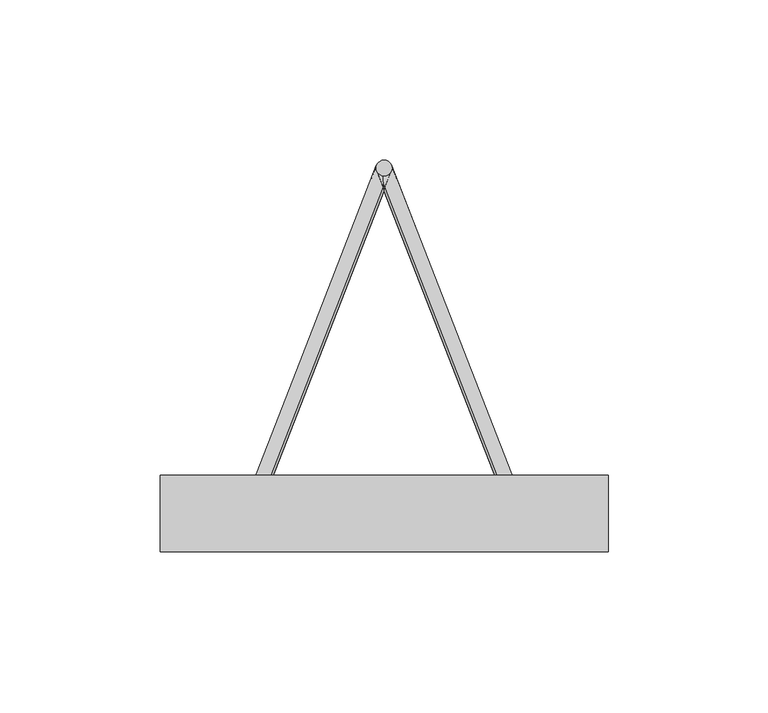
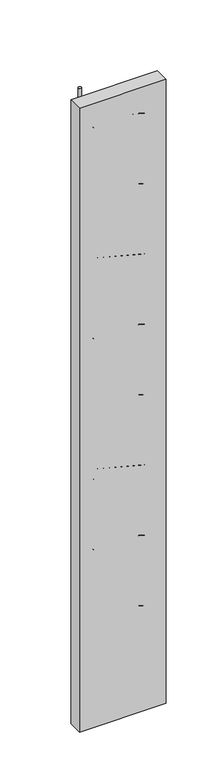
"""IFC4 building model written with IfcOpenShell, lengths in millimetres: proxy geometry, Vigota 4 (Pano 6) (Mf = 85)."""

from ifc_helpers import new_model, si_unit, point, frame, frame_2d, origin, origin_with_axes, origin_2d, place, context, project, spatial, polyline, circle_curve, trimmed, segment, composite_curve, outline, extrude, source, transform, mapped, element, save


def structural_framing_46c3b547(model_context):
    return source(origin(), model_context, "Body", "SweptSolid", [
        extrude(outline(polyline([(-70.0, 12.0), (70.0, 12.0), (70.0, -12.0), (-70.0, -12.0), (-70.0, 12.0)])), origin_with_axes(), (0.0, 0.0, 1.0), 1065.0),
        extrude(outline(composite_curve([segment(trimmed(circle_curve(frame_2d((42.0, 0.0)), 2.5), [point((44.5, 0.0))], [point((39.5, 0.0))], False, "CARTESIAN"), True, "CONTINUOUS"), segment(trimmed(circle_curve(frame_2d((42.0, 0.0)), 2.5), [point((39.5, 0.0))], [point((44.5, 0.0))], False, "CARTESIAN"), True, "CONTINUOUS")], self_intersect=False)), frame((0.0, 0.0, 28.0), z_axis=(0.0, 0.0, 1.0), x_axis=(1.0, 0.0, 0.0)), (0.0, 0.0, 1.0), 1009.0),
        extrude(outline(composite_curve([segment(trimmed(circle_curve(frame_2d((0.0, 108.0)), 2.5), [point((2.5, 108.0))], [point((-2.5, 108.0))], False, "CARTESIAN"), True, "CONTINUOUS"), segment(trimmed(circle_curve(frame_2d((0.0, 108.0)), 2.5), [point((-2.5, 108.0))], [point((2.5, 108.0))], False, "CARTESIAN"), True, "CONTINUOUS")], self_intersect=False)), frame((0.0, 0.0, 62.5), z_axis=(0.0, 0.0, 1.0), x_axis=(1.0, 0.0, 0.0)), (0.0, 0.0, 1.0), 940.0),
        extrude(outline(composite_curve([segment(trimmed(circle_curve(origin_2d(), 2.5), [point((2.5, 0.0))], [point((-2.5, 0.0))], False, "CARTESIAN"), True, "CONTINUOUS"), segment(trimmed(circle_curve(origin_2d(), 2.5), [point((-2.5, 0.0))], [point((2.5, 0.0))], False, "CARTESIAN"), True, "CONTINUOUS")], self_intersect=False)), frame((42.0, 0.0, 52.5), z_axis=(-0.3218603428886276, 0.8276408817707567, 0.4598004898837537), x_axis=(0.8192319205108605, -3.936835275445103e-11, 0.5734623443750141)), (0.0, 0.0, 1.0), 130.491379),
        extrude(outline(composite_curve([segment(trimmed(circle_curve(origin_2d(), 2.5), [point((2.5, 0.0))], [point((-2.5, 0.0))], False, "CARTESIAN"), True, "CONTINUOUS"), segment(trimmed(circle_curve(origin_2d(), 2.5), [point((-2.5, 0.0))], [point((2.5, 0.0))], False, "CARTESIAN"), True, "CONTINUOUS")], self_intersect=False)), frame((0.0, 108.0, 112.5), z_axis=(0.3218603428886276, -0.8276408817707567, 0.4598004898837537), x_axis=(0.8192319205108605, -3.936835275445103e-11, -0.5734623443750141)), (0.0, 0.0, 1.0), 130.491379),
        extrude(outline(composite_curve([segment(trimmed(circle_curve(origin_2d(), 2.5), [point((2.5, 0.0))], [point((-2.5, 0.0))], False, "CARTESIAN"), True, "CONTINUOUS"), segment(trimmed(circle_curve(origin_2d(), 2.5), [point((-2.5, 0.0))], [point((2.5, 0.0))], False, "CARTESIAN"), True, "CONTINUOUS")], self_intersect=False)), frame((42.0, 0.0, 172.5), z_axis=(-0.3218603428886276, 0.8276408817707567, 0.4598004898837537), x_axis=(0.8192319205108605, -3.936835275445103e-11, 0.5734623443750141)), (0.0, 0.0, 1.0), 130.491379),
        extrude(outline(composite_curve([segment(trimmed(circle_curve(origin_2d(), 2.5), [point((2.5, 0.0))], [point((-2.5, 0.0))], False, "CARTESIAN"), True, "CONTINUOUS"), segment(trimmed(circle_curve(origin_2d(), 2.5), [point((-2.5, 0.0))], [point((2.5, 0.0))], False, "CARTESIAN"), True, "CONTINUOUS")], self_intersect=False)), frame((0.0, 108.0, 232.5), z_axis=(0.3218603428886276, -0.8276408817707567, 0.4598004898837537), x_axis=(0.8192319205108605, -3.936835275445103e-11, -0.5734623443750141)), (0.0, 0.0, 1.0), 130.491379),
        extrude(outline(composite_curve([segment(trimmed(circle_curve(origin_2d(), 2.5), [point((2.5, 0.0))], [point((-2.5, 0.0))], False, "CARTESIAN"), True, "CONTINUOUS"), segment(trimmed(circle_curve(origin_2d(), 2.5), [point((-2.5, 0.0))], [point((2.5, 0.0))], False, "CARTESIAN"), True, "CONTINUOUS")], self_intersect=False)), frame((42.0, 0.0, 292.5), z_axis=(-0.3218603428886276, 0.8276408817707567, 0.4598004898837537), x_axis=(0.8192319205108605, -3.936835275445103e-11, 0.5734623443750141)), (0.0, 0.0, 1.0), 130.491379),
        extrude(outline(composite_curve([segment(trimmed(circle_curve(origin_2d(), 2.5), [point((2.5, 0.0))], [point((-2.5, 0.0))], False, "CARTESIAN"), True, "CONTINUOUS"), segment(trimmed(circle_curve(origin_2d(), 2.5), [point((-2.5, 0.0))], [point((2.5, 0.0))], False, "CARTESIAN"), True, "CONTINUOUS")], self_intersect=False)), frame((0.0, 108.0, 352.5), z_axis=(0.3218603428886276, -0.8276408817707567, 0.4598004898837537), x_axis=(0.8192319205108605, -3.936835275445103e-11, -0.5734623443750141)), (0.0, 0.0, 1.0), 130.491379),
        extrude(outline(composite_curve([segment(trimmed(circle_curve(origin_2d(), 2.5), [point((2.5, 0.0))], [point((-2.5, 0.0))], False, "CARTESIAN"), True, "CONTINUOUS"), segment(trimmed(circle_curve(origin_2d(), 2.5), [point((-2.5, 0.0))], [point((2.5, 0.0))], False, "CARTESIAN"), True, "CONTINUOUS")], self_intersect=False)), frame((42.0, 0.0, 412.5), z_axis=(-0.3218603428886276, 0.8276408817707567, 0.4598004898837537), x_axis=(0.8192319205108605, -3.936835275445103e-11, 0.5734623443750141)), (0.0, 0.0, 1.0), 130.491379),
        extrude(outline(composite_curve([segment(trimmed(circle_curve(origin_2d(), 2.5), [point((2.5, 0.0))], [point((-2.5, 0.0))], False, "CARTESIAN"), True, "CONTINUOUS"), segment(trimmed(circle_curve(origin_2d(), 2.5), [point((-2.5, 0.0))], [point((2.5, 0.0))], False, "CARTESIAN"), True, "CONTINUOUS")], self_intersect=False)), frame((0.0, 108.0, 472.5), z_axis=(0.3218603428886276, -0.8276408817707567, 0.4598004898837537), x_axis=(0.8192319205108605, -3.936835275445103e-11, -0.5734623443750141)), (0.0, 0.0, 1.0), 130.491379),
        extrude(outline(composite_curve([segment(trimmed(circle_curve(origin_2d(), 2.5), [point((2.5, 0.0))], [point((-2.5, 0.0))], False, "CARTESIAN"), True, "CONTINUOUS"), segment(trimmed(circle_curve(origin_2d(), 2.5), [point((-2.5, 0.0))], [point((2.5, 0.0))], False, "CARTESIAN"), True, "CONTINUOUS")], self_intersect=False)), frame((42.0, 0.0, 532.5), z_axis=(-0.3218603428886276, 0.8276408817707567, 0.4598004898837537), x_axis=(0.8192319205108605, -3.936835275445103e-11, 0.5734623443750141)), (0.0, 0.0, 1.0), 130.491379),
        extrude(outline(composite_curve([segment(trimmed(circle_curve(origin_2d(), 2.5), [point((2.5, 0.0))], [point((-2.5, 0.0))], False, "CARTESIAN"), True, "CONTINUOUS"), segment(trimmed(circle_curve(origin_2d(), 2.5), [point((-2.5, 0.0))], [point((2.5, 0.0))], False, "CARTESIAN"), True, "CONTINUOUS")], self_intersect=False)), frame((0.0, 108.0, 592.5), z_axis=(0.3218603428886276, -0.8276408817707567, 0.4598004898837537), x_axis=(0.8192319205108605, -3.936835275445103e-11, -0.5734623443750141)), (0.0, 0.0, 1.0), 130.491379),
        extrude(outline(composite_curve([segment(trimmed(circle_curve(origin_2d(), 2.5), [point((2.5, 0.0))], [point((-2.5, 0.0))], False, "CARTESIAN"), True, "CONTINUOUS"), segment(trimmed(circle_curve(origin_2d(), 2.5), [point((-2.5, 0.0))], [point((2.5, 0.0))], False, "CARTESIAN"), True, "CONTINUOUS")], self_intersect=False)), frame((42.0, 0.0, 652.5), z_axis=(-0.3218603428886276, 0.8276408817707567, 0.4598004898837537), x_axis=(0.8192319205108605, -3.936835275445103e-11, 0.5734623443750141)), (0.0, 0.0, 1.0), 130.491379),
        extrude(outline(composite_curve([segment(trimmed(circle_curve(origin_2d(), 2.5), [point((2.5, 0.0))], [point((-2.5, 0.0))], False, "CARTESIAN"), True, "CONTINUOUS"), segment(trimmed(circle_curve(origin_2d(), 2.5), [point((-2.5, 0.0))], [point((2.5, 0.0))], False, "CARTESIAN"), True, "CONTINUOUS")], self_intersect=False)), frame((0.0, 108.0, 712.5), z_axis=(0.3218603428886276, -0.8276408817707567, 0.4598004898837537), x_axis=(0.8192319205108605, -3.936835275445103e-11, -0.5734623443750141)), (0.0, 0.0, 1.0), 130.491379),
        extrude(outline(composite_curve([segment(trimmed(circle_curve(origin_2d(), 2.5), [point((2.5, 0.0))], [point((-2.5, 0.0))], False, "CARTESIAN"), True, "CONTINUOUS"), segment(trimmed(circle_curve(origin_2d(), 2.5), [point((-2.5, 0.0))], [point((2.5, 0.0))], False, "CARTESIAN"), True, "CONTINUOUS")], self_intersect=False)), frame((42.0, 0.0, 772.5), z_axis=(-0.3218603428886276, 0.8276408817707567, 0.4598004898837537), x_axis=(0.8192319205108605, -3.936835275445103e-11, 0.5734623443750141)), (0.0, 0.0, 1.0), 130.491379),
        extrude(outline(composite_curve([segment(trimmed(circle_curve(origin_2d(), 2.5), [point((2.5, 0.0))], [point((-2.5, 0.0))], False, "CARTESIAN"), True, "CONTINUOUS"), segment(trimmed(circle_curve(origin_2d(), 2.5), [point((-2.5, 0.0))], [point((2.5, 0.0))], False, "CARTESIAN"), True, "CONTINUOUS")], self_intersect=False)), frame((0.0, 108.0, 832.5), z_axis=(0.3218603428886276, -0.8276408817707567, 0.4598004898837537), x_axis=(0.8192319205108605, -3.936835275445103e-11, -0.5734623443750141)), (0.0, 0.0, 1.0), 130.491379),
        extrude(outline(composite_curve([segment(trimmed(circle_curve(origin_2d(), 2.5), [point((2.5, 0.0))], [point((-2.5, 0.0))], False, "CARTESIAN"), True, "CONTINUOUS"), segment(trimmed(circle_curve(origin_2d(), 2.5), [point((-2.5, 0.0))], [point((2.5, 0.0))], False, "CARTESIAN"), True, "CONTINUOUS")], self_intersect=False)), frame((42.0, 0.0, 892.5), z_axis=(-0.3218603428886276, 0.8276408817707567, 0.4598004898837537), x_axis=(0.8192319205108605, -3.936835275445103e-11, 0.5734623443750141)), (0.0, 0.0, 1.0), 130.491379),
        extrude(outline(composite_curve([segment(trimmed(circle_curve(origin_2d(), 2.5), [point((2.5, 0.0))], [point((-2.5, 0.0))], False, "CARTESIAN"), True, "CONTINUOUS"), segment(trimmed(circle_curve(origin_2d(), 2.5), [point((-2.5, 0.0))], [point((2.5, 0.0))], False, "CARTESIAN"), True, "CONTINUOUS")], self_intersect=False)), frame((0.0, 108.0, 952.5), z_axis=(0.3218603428886276, -0.8276408817707567, 0.4598004898837537), x_axis=(0.8192319205108605, -3.936835275445103e-11, -0.5734623443750141)), (0.0, 0.0, 1.0), 130.491379),
        extrude(outline(composite_curve([segment(trimmed(circle_curve(frame_2d((-42.0, 0.0)), 2.5), [point((-39.5, 0.0))], [point((-44.5, 0.0))], False, "CARTESIAN"), True, "CONTINUOUS"), segment(trimmed(circle_curve(frame_2d((-42.0, 0.0)), 2.5), [point((-44.5, 0.0))], [point((-39.5, 0.0))], False, "CARTESIAN"), True, "CONTINUOUS")], self_intersect=False)), frame((0.0, 0.0, 28.0), z_axis=(0.0, 0.0, 1.0), x_axis=(1.0, 0.0, 0.0)), (0.0, 0.0, 1.0), 1009.0),
        extrude(outline(composite_curve([segment(trimmed(circle_curve(origin_2d(), 2.5), [point((2.5, 0.0))], [point((-2.5, 0.0))], False, "CARTESIAN"), True, "CONTINUOUS"), segment(trimmed(circle_curve(origin_2d(), 2.5), [point((-2.5, 0.0))], [point((2.5, 0.0))], False, "CARTESIAN"), True, "CONTINUOUS")], self_intersect=False)), frame((-42.0, 0.0, 52.5), z_axis=(0.3218603428886276, 0.8276408817707567, 0.4598004898837537), x_axis=(0.8192319205108605, 3.936835275445103e-11, -0.5734623443750141)), (0.0, 0.0, 1.0), 130.491379),
        extrude(outline(composite_curve([segment(trimmed(circle_curve(origin_2d(), 2.5), [point((2.5, 0.0))], [point((-2.5, 0.0))], False, "CARTESIAN"), True, "CONTINUOUS"), segment(trimmed(circle_curve(origin_2d(), 2.5), [point((-2.5, 0.0))], [point((2.5, 0.0))], False, "CARTESIAN"), True, "CONTINUOUS")], self_intersect=False)), frame((0.0, 108.0, 112.5), z_axis=(-0.3218603428886276, -0.8276408817707567, 0.4598004898837537), x_axis=(0.8192319205108605, 3.936835275445103e-11, 0.5734623443750141)), (0.0, 0.0, 1.0), 130.491379),
        extrude(outline(composite_curve([segment(trimmed(circle_curve(origin_2d(), 2.5), [point((2.5, 0.0))], [point((-2.5, 0.0))], False, "CARTESIAN"), True, "CONTINUOUS"), segment(trimmed(circle_curve(origin_2d(), 2.5), [point((-2.5, 0.0))], [point((2.5, 0.0))], False, "CARTESIAN"), True, "CONTINUOUS")], self_intersect=False)), frame((-42.0, 0.0, 172.5), z_axis=(0.3218603428886276, 0.8276408817707567, 0.4598004898837537), x_axis=(0.8192319205108605, 3.936835275445103e-11, -0.5734623443750141)), (0.0, 0.0, 1.0), 130.491379),
        extrude(outline(composite_curve([segment(trimmed(circle_curve(origin_2d(), 2.5), [point((2.5, 0.0))], [point((-2.5, 0.0))], False, "CARTESIAN"), True, "CONTINUOUS"), segment(trimmed(circle_curve(origin_2d(), 2.5), [point((-2.5, 0.0))], [point((2.5, 0.0))], False, "CARTESIAN"), True, "CONTINUOUS")], self_intersect=False)), frame((0.0, 108.0, 232.5), z_axis=(-0.3218603428886276, -0.8276408817707567, 0.4598004898837537), x_axis=(0.8192319205108605, 3.936835275445103e-11, 0.5734623443750141)), (0.0, 0.0, 1.0), 130.491379),
        extrude(outline(composite_curve([segment(trimmed(circle_curve(origin_2d(), 2.5), [point((2.5, 0.0))], [point((-2.5, 0.0))], False, "CARTESIAN"), True, "CONTINUOUS"), segment(trimmed(circle_curve(origin_2d(), 2.5), [point((-2.5, 0.0))], [point((2.5, 0.0))], False, "CARTESIAN"), True, "CONTINUOUS")], self_intersect=False)), frame((-42.0, 0.0, 292.5), z_axis=(0.3218603428886276, 0.8276408817707567, 0.4598004898837537), x_axis=(0.8192319205108605, 3.936835275445103e-11, -0.5734623443750141)), (0.0, 0.0, 1.0), 130.491379),
        extrude(outline(composite_curve([segment(trimmed(circle_curve(origin_2d(), 2.5), [point((2.5, 0.0))], [point((-2.5, 0.0))], False, "CARTESIAN"), True, "CONTINUOUS"), segment(trimmed(circle_curve(origin_2d(), 2.5), [point((-2.5, 0.0))], [point((2.5, 0.0))], False, "CARTESIAN"), True, "CONTINUOUS")], self_intersect=False)), frame((0.0, 108.0, 352.5), z_axis=(-0.3218603428886276, -0.8276408817707567, 0.4598004898837537), x_axis=(0.8192319205108605, 3.936835275445103e-11, 0.5734623443750141)), (0.0, 0.0, 1.0), 130.491379),
        extrude(outline(composite_curve([segment(trimmed(circle_curve(origin_2d(), 2.5), [point((2.5, 0.0))], [point((-2.5, 0.0))], False, "CARTESIAN"), True, "CONTINUOUS"), segment(trimmed(circle_curve(origin_2d(), 2.5), [point((-2.5, 0.0))], [point((2.5, 0.0))], False, "CARTESIAN"), True, "CONTINUOUS")], self_intersect=False)), frame((-42.0, 0.0, 412.5), z_axis=(0.3218603428886276, 0.8276408817707567, 0.4598004898837537), x_axis=(0.8192319205108605, 3.936835275445103e-11, -0.5734623443750141)), (0.0, 0.0, 1.0), 130.491379),
        extrude(outline(composite_curve([segment(trimmed(circle_curve(origin_2d(), 2.5), [point((2.5, 0.0))], [point((-2.5, 0.0))], False, "CARTESIAN"), True, "CONTINUOUS"), segment(trimmed(circle_curve(origin_2d(), 2.5), [point((-2.5, 0.0))], [point((2.5, 0.0))], False, "CARTESIAN"), True, "CONTINUOUS")], self_intersect=False)), frame((0.0, 108.0, 472.5), z_axis=(-0.3218603428886276, -0.8276408817707567, 0.4598004898837537), x_axis=(0.8192319205108605, 3.936835275445103e-11, 0.5734623443750141)), (0.0, 0.0, 1.0), 130.491379),
        extrude(outline(composite_curve([segment(trimmed(circle_curve(origin_2d(), 2.5), [point((2.5, 0.0))], [point((-2.5, 0.0))], False, "CARTESIAN"), True, "CONTINUOUS"), segment(trimmed(circle_curve(origin_2d(), 2.5), [point((-2.5, 0.0))], [point((2.5, 0.0))], False, "CARTESIAN"), True, "CONTINUOUS")], self_intersect=False)), frame((-42.0, 0.0, 532.5), z_axis=(0.3218603428886276, 0.8276408817707567, 0.4598004898837537), x_axis=(0.8192319205108605, 3.936835275445103e-11, -0.5734623443750141)), (0.0, 0.0, 1.0), 130.491379),
        extrude(outline(composite_curve([segment(trimmed(circle_curve(origin_2d(), 2.5), [point((2.5, 0.0))], [point((-2.5, 0.0))], False, "CARTESIAN"), True, "CONTINUOUS"), segment(trimmed(circle_curve(origin_2d(), 2.5), [point((-2.5, 0.0))], [point((2.5, 0.0))], False, "CARTESIAN"), True, "CONTINUOUS")], self_intersect=False)), frame((0.0, 108.0, 592.5), z_axis=(-0.3218603428886276, -0.8276408817707567, 0.4598004898837537), x_axis=(0.8192319205108605, 3.936835275445103e-11, 0.5734623443750141)), (0.0, 0.0, 1.0), 130.491379),
        extrude(outline(composite_curve([segment(trimmed(circle_curve(origin_2d(), 2.5), [point((2.5, 0.0))], [point((-2.5, 0.0))], False, "CARTESIAN"), True, "CONTINUOUS"), segment(trimmed(circle_curve(origin_2d(), 2.5), [point((-2.5, 0.0))], [point((2.5, 0.0))], False, "CARTESIAN"), True, "CONTINUOUS")], self_intersect=False)), frame((-42.0, 0.0, 652.5), z_axis=(0.3218603428886276, 0.8276408817707567, 0.4598004898837537), x_axis=(0.8192319205108605, 3.936835275445103e-11, -0.5734623443750141)), (0.0, 0.0, 1.0), 130.491379),
        extrude(outline(composite_curve([segment(trimmed(circle_curve(origin_2d(), 2.5), [point((2.5, 0.0))], [point((-2.5, 0.0))], False, "CARTESIAN"), True, "CONTINUOUS"), segment(trimmed(circle_curve(origin_2d(), 2.5), [point((-2.5, 0.0))], [point((2.5, 0.0))], False, "CARTESIAN"), True, "CONTINUOUS")], self_intersect=False)), frame((0.0, 108.0, 712.5), z_axis=(-0.3218603428886276, -0.8276408817707567, 0.4598004898837537), x_axis=(0.8192319205108605, 3.936835275445103e-11, 0.5734623443750141)), (0.0, 0.0, 1.0), 130.491379),
        extrude(outline(composite_curve([segment(trimmed(circle_curve(origin_2d(), 2.5), [point((2.5, 0.0))], [point((-2.5, 0.0))], False, "CARTESIAN"), True, "CONTINUOUS"), segment(trimmed(circle_curve(origin_2d(), 2.5), [point((-2.5, 0.0))], [point((2.5, 0.0))], False, "CARTESIAN"), True, "CONTINUOUS")], self_intersect=False)), frame((-42.0, 0.0, 772.5), z_axis=(0.3218603428886276, 0.8276408817707567, 0.4598004898837537), x_axis=(0.8192319205108605, 3.936835275445103e-11, -0.5734623443750141)), (0.0, 0.0, 1.0), 130.491379),
        extrude(outline(composite_curve([segment(trimmed(circle_curve(origin_2d(), 2.5), [point((2.5, 0.0))], [point((-2.5, 0.0))], False, "CARTESIAN"), True, "CONTINUOUS"), segment(trimmed(circle_curve(origin_2d(), 2.5), [point((-2.5, 0.0))], [point((2.5, 0.0))], False, "CARTESIAN"), True, "CONTINUOUS")], self_intersect=False)), frame((0.0, 108.0, 832.5), z_axis=(-0.3218603428886276, -0.8276408817707567, 0.4598004898837537), x_axis=(0.8192319205108605, 3.936835275445103e-11, 0.5734623443750141)), (0.0, 0.0, 1.0), 130.491379),
        extrude(outline(composite_curve([segment(trimmed(circle_curve(origin_2d(), 2.5), [point((2.5, 0.0))], [point((-2.5, 0.0))], False, "CARTESIAN"), True, "CONTINUOUS"), segment(trimmed(circle_curve(origin_2d(), 2.5), [point((-2.5, 0.0))], [point((2.5, 0.0))], False, "CARTESIAN"), True, "CONTINUOUS")], self_intersect=False)), frame((-42.0, 0.0, 892.5), z_axis=(0.3218603428886276, 0.8276408817707567, 0.4598004898837537), x_axis=(0.8192319205108605, 3.936835275445103e-11, -0.5734623443750141)), (0.0, 0.0, 1.0), 130.491379),
        extrude(outline(composite_curve([segment(trimmed(circle_curve(origin_2d(), 2.5), [point((2.5, 0.0))], [point((-2.5, 0.0))], False, "CARTESIAN"), True, "CONTINUOUS"), segment(trimmed(circle_curve(origin_2d(), 2.5), [point((-2.5, 0.0))], [point((2.5, 0.0))], False, "CARTESIAN"), True, "CONTINUOUS")], self_intersect=False)), frame((0.0, 108.0, 952.5), z_axis=(-0.3218603428886276, -0.8276408817707567, 0.4598004898837537), x_axis=(0.8192319205108605, 3.936835275445103e-11, 0.5734623443750141)), (0.0, 0.0, 1.0), 130.491379),
    ])


if __name__ == "__main__":
    model = new_model("IFC4")
    model_context = context("Model", 3, world=origin())
    ifc_project = project(units=[si_unit("LENGTHUNIT", "METRE", prefix="MILLI")], contexts=[model_context])
    site = spatial("IfcSite", under=ifc_project)
    building = spatial("IfcBuilding", under=site)
    placement = place(None, origin())
    structural_framing_shape = structural_framing_46c3b547(model_context)
    element("IfcBuildingElementProxy", 1, Name="Vigota 4 (Pano 6) (Mf = 85)", ObjectType="Vigota 4 (Pano 6) (Mf = 85)", at=placement, inside=building, context=model_context, shape_type="MappedRepresentation", body=[
        mapped(structural_framing_shape, transform((0.0, 0.0, 0.0), x_axis=(1.0, 0.0, 0.0), y_axis=(0.0, 1.0, 0.0), z_axis=(0.0, 0.0, 1.0))),
    ])
    save(model, "model.ifc")

# Revit data of these elements
# Element 1 (IfcBuildingElementProxy, "Vigota 4 (Pano 6) (Mf = 85)")
#   Materials on its faces: "Aço", "Concreto armado"
# Materials
#   "Aço": class "Metal", colour RGB 120 120 120, transparency 0, Description = "Aço estrutural A36 grau, ASTM B, acabamento laminado", Cost = 0
#   "Concreto armado": class "Não atribuído", colour RGB 168 169 158, transparency 0
